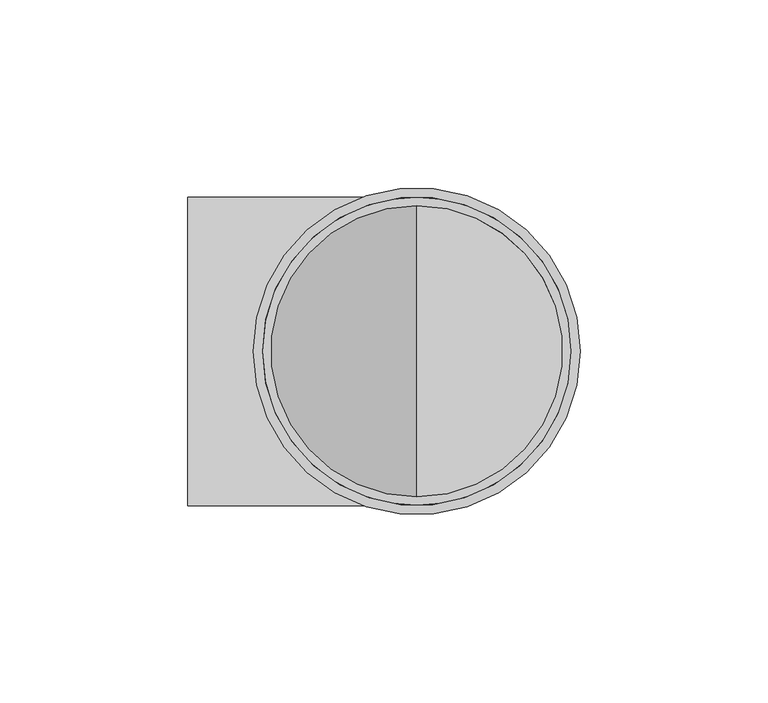
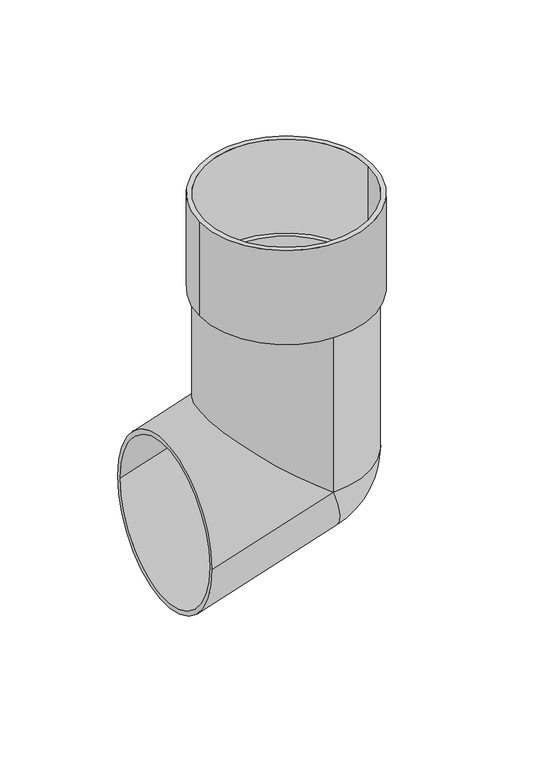
"""IFC4 building model written with IfcOpenShell, lengths in millimetres: proxy geometry, ⇲ Водосточный слив с хомутом крепления трубы : ⇲ Водосточный слив с хомутом крепления трубы."""

import ifcopenshell
import ifcopenshell.guid

model = None  # the IFC model being written
_history = None  # IfcOwnerHistory: only IFC2X3 demands one
_inside = {}  # id of a spatial element -> (the spatial element, [elements in it])
_under = {}  # id of a project, library or spatial element -> (it, [spatial elements below it])
_declared = {}  # id of a project -> (the project, [libraries it declares])
_typed = {}  # id of a type object -> (the type object, [elements of that type])
_made_of = {}  # id of a material, layer set ... -> (it, [elements and type objects made of it])


def new_model(schema):
    """Start an empty IFC model of exactly this schema.

    Asked for "IFC4X3", IfcOpenShell would pick the latest addendum, in which some entities
    have other attributes; the version numbers below select the first issue.
    IFC2X3 requires an IfcOwnerHistory on every rooted entity: one is made here for all.
    """
    global model, _history
    if schema == "IFC4X3":
        model = ifcopenshell.file(schema_version=(4, 3, 0, 0))
    else:
        model = ifcopenshell.file(schema=schema)
    _inside.clear()
    _under.clear()
    _declared.clear()
    _typed.clear()
    _made_of.clear()
    _history = None
    if model.schema == "IFC2X3":
        org = make("IfcOrganization", Name="unknown")
        user = make(
            "IfcPersonAndOrganization",
            ThePerson=make("IfcPerson", FamilyName="unknown"),
            TheOrganization=org,
        )
        app = make(
            "IfcApplication",
            ApplicationDeveloper=org,
            Version="unknown",
            ApplicationFullName="unknown",
            ApplicationIdentifier="unknown",
        )
        _history = make(
            "IfcOwnerHistory",
            OwningUser=user,
            OwningApplication=app,
            ChangeAction="ADDED",
            CreationDate=0,
        )
    return model


def make(cls, **values):
    """One entity of the class cls with the attributes given. An attribute that is None is left unset."""
    return model.create_entity(
        cls, **{name: value for name, value in values.items() if value is not None}
    )


def rooted(cls, **values):
    """An entity with a GlobalId (a new one), such as an element, a storey or a relation."""
    return make(cls, GlobalId=ifcopenshell.guid.new(), OwnerHistory=_history, **values)


def si_unit(unit_type, name, prefix=None):
    """IfcSIUnit, for example si_unit("LENGTHUNIT", "METRE", prefix="MILLI")."""
    return make("IfcSIUnit", UnitType=unit_type, Prefix=prefix, Name=name)


def assignment(units):
    """IfcUnitAssignment: the units of a project."""
    return None if units is None else make("IfcUnitAssignment", Units=units)


def point(xyz):
    """IfcCartesianPoint."""
    return None if xyz is None else make("IfcCartesianPoint", Coordinates=xyz)


def direction(xyz):
    """IfcDirection."""
    return None if xyz is None else make("IfcDirection", DirectionRatios=xyz)


def frame(location, z_axis=None, x_axis=None):
    """IfcAxis2Placement3D, a coordinate frame: its origin and axes. An axis left out is left unset."""
    return make(
        "IfcAxis2Placement3D",
        Location=point(location),
        Axis=direction(z_axis),
        RefDirection=direction(x_axis),
    )


def origin():
    """The frame at (0, 0, 0) with its axes left unset."""
    return frame((0.0, 0.0, 0.0))


def origin_with_axes():
    """The frame at (0, 0, 0) with the z axis (0, 0, 1) and the x axis (1, 0, 0) written out."""
    return frame((0.0, 0.0, 0.0), z_axis=(0.0, 0.0, 1.0), x_axis=(1.0, 0.0, 0.0))


def place(relative_to, where):
    """IfcLocalPlacement: puts the frame where relative to a parent placement (None: the world)."""
    return make(
        "IfcLocalPlacement", PlacementRelTo=relative_to, RelativePlacement=where
    )


def context(
    kind, dimensions, precision=None, world=None, true_north=None, identifier=None
):
    """IfcGeometricRepresentationContext, for example the 3D "Model" context."""
    return make(
        "IfcGeometricRepresentationContext",
        ContextIdentifier=identifier,
        ContextType=kind,
        CoordinateSpaceDimension=dimensions,
        Precision=precision,
        WorldCoordinateSystem=world,
        TrueNorth=true_north,
    )


def project(units=None, contexts=None):
    """IfcProject with its units and contexts."""
    return rooted(
        "IfcProject",
        Name="project",
        RepresentationContexts=contexts,
        UnitsInContext=assignment(units),
    )


def spatial(cls, under=None, at=None, **own):
    """A site, building, storey or space (cls), placed at a placement, below another one or the project."""
    s = rooted(cls, ObjectPlacement=at, **own)
    if under is not None:
        _under.setdefault(under.id(), (under, []))[1].append(s)
    return s


def polyline(points):
    """IfcPolyline through the points."""
    return make("IfcPolyline", Points=[point(p) for p in points])


def circle_curve(where, radius):
    """IfcCircle in the frame where."""
    return make("IfcCircle", Position=where, Radius=radius)


def ellipse_curve(where, semi_axis1, semi_axis2):
    """IfcEllipse in the frame where."""
    return make(
        "IfcEllipse", Position=where, SemiAxis1=semi_axis1, SemiAxis2=semi_axis2
    )


def trimmed(basis, trim1, trim2, sense, master):
    """IfcTrimmedCurve: the piece of a basis curve between two trims."""
    return make(
        "IfcTrimmedCurve",
        BasisCurve=basis,
        Trim1=trim1,
        Trim2=trim2,
        SenseAgreement=sense,
        MasterRepresentation=master,
    )


def shape(context_of_items, identifier, shape_type, items):
    """IfcShapeRepresentation: the items that make up one representation, for example the "Body"."""
    return make(
        "IfcShapeRepresentation",
        ContextOfItems=context_of_items,
        RepresentationIdentifier=identifier,
        RepresentationType=shape_type,
        Items=items,
    )


def source(mapping_origin, context_of_items, identifier, shape_type, items):
    """IfcRepresentationMap: a shape defined once, which mapped items show again and again."""
    return make(
        "IfcRepresentationMap",
        MappingOrigin=mapping_origin,
        MappedRepresentation=shape(context_of_items, identifier, shape_type, items),
    )


def transform(
    local_origin,
    x_axis=None,
    y_axis=None,
    z_axis=None,
    scale=None,
    scale2=None,
    scale3=None,
    uniform=True,
):
    """IfcCartesianTransformationOperator3D, or its non-uniform kind. x_axis, y_axis, z_axis: its Axis1, 2, 3."""
    if uniform:
        return make(
            "IfcCartesianTransformationOperator3D",
            Axis1=direction(x_axis),
            Axis2=direction(y_axis),
            LocalOrigin=point(local_origin),
            Scale=scale,
            Axis3=direction(z_axis),
        )
    return make(
        "IfcCartesianTransformationOperator3DnonUniform",
        Axis1=direction(x_axis),
        Axis2=direction(y_axis),
        LocalOrigin=point(local_origin),
        Scale=scale,
        Axis3=direction(z_axis),
        Scale2=scale2,
        Scale3=scale3,
    )


def mapped(mapping_source, mapping_target):
    """IfcMappedItem: shows the shape of a source again, moved by a transform."""
    return make(
        "IfcMappedItem", MappingSource=mapping_source, MappingTarget=mapping_target
    )


def made_of(thing, what):
    """Note that an element or type object is made of a material, layer set ...; save() writes the relation."""
    if what is not None:
        _made_of.setdefault(what.id(), (what, []))[1].append(thing)
    return thing


def element(
    cls,
    number,
    at=None,
    inside=None,
    cuts=None,
    type_object=None,
    material=None,
    context=None,
    identifier="Body",
    shape_type=None,
    held_by="IfcProductDefinitionShape",
    body=None,
    shapes=None,
    **own,
):
    """One element of the class cls, such as IfcWall. Its Tag is "e" and its number.

    at: its placement. inside: the storey or other place that contains it. cuts: it is an
    opening in that element (IfcRelVoidsElement). A single representation is given by context,
    identifier, shape_type and body (its items); several are given by shapes. held_by: the class
    of the entity that holds the representations. save() writes the other relations.
    """
    e = rooted(cls, Tag="e%d" % number, ObjectPlacement=at, **own)
    if body is not None:
        shapes = [shape(context, identifier, shape_type, body)]
    if shapes is not None:
        e.Representation = make(held_by, Representations=shapes)
    if inside is not None:
        _inside.setdefault(inside.id(), (inside, []))[1].append(e)
    if cuts is not None:
        rooted(
            "IfcRelVoidsElement", RelatingBuildingElement=cuts, RelatedOpeningElement=e
        )
    if type_object is not None:
        _typed.setdefault(type_object.id(), (type_object, []))[1].append(e)
    return made_of(e, material)


def aggregate(whole, parts):
    """IfcRelAggregates: a whole, such as a stair, and the parts it consists of."""
    return rooted("IfcRelAggregates", RelatingObject=whole, RelatedObjects=parts)


def save(model, path):
    """Write the relations noted so far, then the file.

    IfcRelAggregates (storeys below a building ...), IfcRelContainedInSpatialStructure (elements
    in a storey), IfcRelDefinesByType, IfcRelAssociatesMaterial and IfcRelDeclares: one each for
    every whole, place, type object, material and project.
    """
    for whole, parts in _under.values():
        aggregate(whole, parts)
    for where, things in _inside.values():
        rooted(
            "IfcRelContainedInSpatialStructure",
            RelatedElements=things,
            RelatingStructure=where,
        )
    for kind, things in _typed.values():
        rooted("IfcRelDefinesByType", RelatedObjects=things, RelatingType=kind)
    for what, things in _made_of.values():
        rooted("IfcRelAssociatesMaterial", RelatedObjects=things, RelatingMaterial=what)
    for by, libraries in _declared.values():
        rooted("IfcRelDeclares", RelatingContext=by, RelatedDefinitions=libraries)
    model.write(path)


def plane_surface(at):
    """IfcPlane: the flat surface through the origin of the frame at, square to its z axis."""
    return make("IfcPlane", Position=at)


def cylinder_surface(at, radius):
    """IfcCylindricalSurface: all points at the distance radius from the z axis of the frame at."""
    return make("IfcCylindricalSurface", Position=at, Radius=radius)


def revolved_surface(curve, axis_point, axis_direction):
    """IfcSurfaceOfRevolution: the curve turned about the line through axis_point along axis_direction."""
    return make(
        "IfcSurfaceOfRevolution",
        SweptCurve=make("IfcArbitraryOpenProfileDef", ProfileType="CURVE", Curve=curve),
        AxisPosition=make("IfcAxis1Placement", Location=point(axis_point), Axis=direction(axis_direction)),
    )


def advanced_brep(points, edges, surfaces, faces):
    """IfcAdvancedBrep: a solid bounded by faces that lie on surfaces and meet in shared edges.

    An edge is (start, end): straight between two places in points (the first is 0);
    or (start, end, curve); or (start, end, curve, False) where it runs against its curve.
    A face is (place in surfaces, loops), or (place, loops, False) where it looks against
    its surface's normal. A loop lists edges by number (the first is 1), with a minus sign
    where the edge is run from its end to its start. The first loop is the outer one.
    """
    corners = [point(p) for p in points]
    vertices = [make("IfcVertexPoint", VertexGeometry=c) for c in corners]
    made = []
    for start, end, *more in edges:
        made.append(
            make(
                "IfcEdgeCurve",
                EdgeStart=vertices[start],
                EdgeEnd=vertices[end],
                EdgeGeometry=more[0] if more else make("IfcPolyline", Points=[corners[start], corners[end]]),
                SameSense=more[1] if len(more) > 1 else True,
            )
        )
    hull = []
    for where, loops, *sense in faces:
        bounds = []
        for j, loop in enumerate(loops):
            ring = [make("IfcOrientedEdge", EdgeElement=made[abs(k) - 1], Orientation=k > 0) for k in loop]
            bounds.append(
                make(
                    "IfcFaceOuterBound" if j == 0 else "IfcFaceBound",
                    Bound=make("IfcEdgeLoop", EdgeList=ring),
                    Orientation=True,
                )
            )
        hull.append(make("IfcAdvancedFace", Bounds=bounds, FaceSurface=surfaces[where], SameSense=sense[0] if sense else True))
    return make("IfcAdvancedBrep", Outer=make("IfcClosedShell", CfsFaces=hull))


def generic_models_fbe01fe8(model_context):
    return source(origin(), model_context, "Body", "AdvancedBrep", [
        advanced_brep(
        [(41.1, 0.0, -50.0), (0.0, 41.1, -50.0), (-41.1, 0.0, -50.0), (0.0, -41.1, -50.0), (0.0, 38.8, -50.0), (0.0, -38.8, -50.0), (0.0, 41.1, -50.0), (0.0, 41.1, -134.0), (0.0, -41.1, -134.0), (0.0, -41.1, -50.0), (-41.1, 0.0, -50.0), (41.1, 0.0, -50.0), (0.0, 38.8, -134.0), (0.0, -38.8, -134.0), (-61.0, 41.1, -153.8201015), (-61.0, -41.1, -153.8201015), (-61.0, 38.8, -153.8201015), (-61.0, -38.8, -153.8201015), (-43.6, 0.0, 0.0), (43.6, 0.0, 0.0), (-41.1, 0.0, 0.0), (41.1, 0.0, 0.0), (-43.6, 0.0, -50.0), (43.6, 0.0, -50.0)],
        [
            (0, 1, circle_curve(frame((0.0, 0.0, -50.0), z_axis=(0.0, 0.0, 1.0), x_axis=(1.0, 0.0, 0.0)), 41.1)),
            (1, 2, circle_curve(frame((0.0, 0.0, -50.0), z_axis=(0.0, 0.0, 1.0), x_axis=(1.0, 0.0, 0.0)), 41.1)),
            (2, 3, circle_curve(frame((0.0, 0.0, -50.0), z_axis=(0.0, 0.0, 1.0), x_axis=(1.0, 0.0, 0.0)), 41.1)),
            (3, 0, circle_curve(frame((0.0, 0.0, -50.0), z_axis=(0.0, 0.0, 1.0), x_axis=(1.0, 0.0, 0.0)), 41.1)),
            (4, 5, circle_curve(frame((0.0, 0.0, -50.0), z_axis=(0.0, 0.0, -1.0), x_axis=(0.0, -1.0, 0.0)), 38.8)),
            (5, 4, circle_curve(frame((0.0, 0.0, -50.0), z_axis=(0.0, 0.0, -1.0), x_axis=(0.0, -1.0, 0.0)), 38.8)),
            (6, 7),
            (7, 8, ellipse_curve(frame((0.0, 0.0, -134.0), z_axis=(0.5877852522924744, 0.0, 0.8090169943749465), x_axis=(-0.8090169943749465, 0.0, 0.5877852522924745)), 50.8023939, 41.1)),
            (8, 9),
            (9, 10, circle_curve(frame((0.0, 0.0, -50.0), z_axis=(0.0, 0.0, -1.0), x_axis=(0.0, -1.0, 0.0)), 41.1)),
            (10, 6, circle_curve(frame((0.0, 0.0, -50.0), z_axis=(0.0, 0.0, -1.0), x_axis=(0.0, -1.0, 0.0)), 41.1)),
            (6, 11, circle_curve(frame((0.0, 0.0, -50.0), z_axis=(0.0, 0.0, -1.0), x_axis=(0.0, -1.0, 0.0)), 41.1)),
            (11, 9, circle_curve(frame((0.0, 0.0, -50.0), z_axis=(0.0, 0.0, -1.0), x_axis=(0.0, -1.0, 0.0)), 41.1)),
            (8, 7, circle_curve(frame((0.0, 0.0, -134.0), z_axis=(0.0, 0.0, 1.0), x_axis=(0.0, -1.0, 0.0)), 41.1)),
            (4, 12),
            (12, 13, circle_curve(frame((0.0, 0.0, -134.0), z_axis=(0.0, 0.0, -1.0), x_axis=(0.0, -1.0, 0.0)), 38.8)),
            (13, 5),
            (13, 12, ellipse_curve(frame((0.0, 0.0, -134.0), z_axis=(-0.5877852522924744, 0.0, -0.8090169943749465), x_axis=(0.8090169943749465, 0.0, -0.5877852522924745)), 47.9594375, 38.8)),
            (7, 14),
            (14, 15, ellipse_curve(frame((-61.0, 0.0, -153.8201015), z_axis=(1.0, 0.0, 0.0), x_axis=(0.0, 0.0, 1.0)), 43.2150974, 41.1)),
            (15, 8),
            (7, 8, circle_curve(frame((0.0, 0.0, -134.0), z_axis=(-0.9510565162951546, 0.0, -0.30901699437494456), x_axis=(0.0, -1.0, 0.0)), 41.1)),
            (15, 14, ellipse_curve(frame((-61.0, 0.0, -153.8201015), z_axis=(1.0, 0.0, 0.0), x_axis=(0.0, 0.0, 1.0)), 43.2150974, 41.1)),
            (13, 12, circle_curve(frame((0.0, 0.0, -134.0), z_axis=(0.9510565162951546, 0.0, 0.30901699437494456), x_axis=(0.0, -1.0, 0.0)), 38.8)),
            (12, 16),
            (16, 17, ellipse_curve(frame((-61.0, 0.0, -153.8201015), z_axis=(-1.0, 0.0, 0.0), x_axis=(0.0, 0.0, -1.0)), 40.7967343, 38.8)),
            (17, 13),
            (17, 16, ellipse_curve(frame((-61.0, 0.0, -153.8201015), z_axis=(-1.0, 0.0, 0.0), x_axis=(0.0, 0.0, -1.0)), 40.7967343, 38.8)),
            (12, 13),
            (18, 19, circle_curve(origin_with_axes(), 43.6)),
            (19, 18, circle_curve(origin_with_axes(), 43.6)),
            (20, 21, circle_curve(frame((0.0, 0.0, 0.0), z_axis=(0.0, 0.0, -1.0), x_axis=(1.0, 0.0, 0.0)), 41.1)),
            (21, 20, circle_curve(frame((0.0, 0.0, 0.0), z_axis=(0.0, 0.0, -1.0), x_axis=(1.0, 0.0, 0.0)), 41.1)),
            (22, 23, circle_curve(frame((0.0, 0.0, -50.0), z_axis=(0.0, 0.0, -1.0), x_axis=(1.0, 0.0, 0.0)), 43.6)),
            (23, 22, circle_curve(frame((0.0, 0.0, -50.0), z_axis=(0.0, 0.0, -1.0), x_axis=(1.0, 0.0, 0.0)), 43.6)),
            (20, 2),
            (0, 21),
            (18, 22),
            (23, 19),
        ],
        [
            plane_surface(frame((0.0, 0.0, -50.0), z_axis=(0.0, 0.0, 1.0), x_axis=(0.0, -1.0, 0.0))),
            cylinder_surface(frame((0.0, 0.0, -50.0), z_axis=(0.0, 0.0, 1.0), x_axis=(0.0, -1.0, 0.0)), 41.1),
            revolved_surface(polyline([(0.0, -38.8, -134.0), (0.0, -38.8, -50.0)]), (0.0, 0.0, -50.0), (0.0, 0.0, -1.0)),
            revolved_surface(polyline([(0.0, -38.8, -162.18985007074266), (0.0, -38.8, -50.0)]), (0.0, 0.0, -50.0), (0.0, 0.0, -1.0)),
            cylinder_surface(frame((0.0, 0.0, -134.0), z_axis=(0.9510565162951546, 0.0, 0.30901699437494456), x_axis=(0.0, -1.0, 0.0)), 41.1),
            revolved_surface(polyline([(-72.98985939037308, -38.8, -157.7158429412023), (0.0, -38.8, -134.0)]), (0.0, 0.0, -134.0), (-0.9510565162951546, 0.0, -0.30901699437494456)),
            revolved_surface(polyline([(-72.98985939037308, -38.8, -157.7158429412023), (26.810140603163227, -38.8, -125.28885725925879)]), (0.0, 0.0, -134.0), (-0.9510565162951546, 0.0, -0.30901699437494456)),
            plane_surface(frame((0.0, 50.0, -134.0), z_axis=(0.0, 0.0, 1.0), x_axis=(1.0, 0.0, 0.0))),
            plane_surface(frame((0.0, 50.0, -134.0), z_axis=(-0.9510565162951546, 0.0, -0.30901699437494445), x_axis=(0.30901699437494445, 0.0, -0.9510565162951546))),
            revolved_surface(trimmed(ellipse_curve(frame((0.0, 0.0, -134.0), z_axis=(0.0, 0.0, 1.0), x_axis=(1.0, 0.0, 0.0)), 41.1, 41.1), [point((0.0, -41.1, -134.0))], [point((0.0, 41.1, -134.0))], True, "CARTESIAN"), (0.0, 50.0, -134.0), (0.0, 1.0, 0.0)),
            plane_surface(frame((41.1, 0.0, 0.0), z_axis=(0.0, 0.0, 1.0), x_axis=(0.0, -1.0, 0.0))),
            plane_surface(frame((41.1, 0.0, -50.0), z_axis=(0.0, 0.0, -1.0), x_axis=(0.0, 1.0, 0.0))),
            revolved_surface(polyline([(41.1, 0.0, -50.0), (41.1, 0.0, 0.0)]), (0.0, 0.0, -50.0), (0.0, 0.0, -1.0)),
            cylinder_surface(origin_with_axes(), 43.6),
            plane_surface(frame((-61.0, -49.4498638, -215.0), z_axis=(-1.0, 0.0, 0.0), x_axis=(0.0, 1.0, 0.0))),
        ],
        [
            (0, [[1, 2, 3, 4], [5, 6]]),
            (1, [[7, 8, 9, 10, 11]]),
            (1, [[-7, 12, 13, -9, 14]]),
            (2, [[-5, 15, 16, 17]]),
            (3, [[-6, -17, 18, -15]]),
            (4, [[-8, 19, 20, 21]]),
            (4, [[22, -21, 23, -19]]),
            (5, [[24, 25, 26, 27]]),
            (6, [[-18, -27, 28, -25]]),
            (7, [[29, -16]]),
            (8, [[-29, -24]]),
            (9, [[-14, -22]]),
            (10, [[30, 31], [32, 33]]),
            (11, [[34, 35], [-11, -10, -13, -12]]),
            (12, [[-32, 36, -2, -1, 37]]),
            (12, [[-33, -37, -4, -3, -36]]),
            (13, [[-30, 38, -35, 39]]),
            (13, [[-31, -39, -34, -38]]),
            (14, [[-20, -23], [-26, -28]]),
        ],
    ),
    ])


if __name__ == "__main__":
    model = new_model("IFC4")
    model_context = context("Model", 3, world=origin())
    ifc_project = project(units=[si_unit("LENGTHUNIT", "METRE", prefix="MILLI")], contexts=[model_context])
    site = spatial("IfcSite", under=ifc_project)
    building = spatial("IfcBuilding", under=site)
    placement = place(None, origin())
    generic_models_shape = generic_models_fbe01fe8(model_context)
    element("IfcBuildingElementProxy", 1, Name="⇲ Водосточный слив с хомутом крепления трубы : ⇲ Водосточный слив с хомутом крепления трубы", ObjectType="⇲ Водосточный слив с хомутом крепления трубы : ⇲ Водосточный слив с хомутом крепления трубы", at=placement, inside=building, context=model_context, shape_type="MappedRepresentation", body=[
        mapped(generic_models_shape, transform((0.0, 0.0, 0.0), x_axis=(1.0, 0.0, 0.0), y_axis=(0.0, 1.0, 0.0), z_axis=(0.0, 0.0, 1.0))),
    ])
    save(model, "model.ifc")

# Revit data of these elements
# Type "⇲ Водосточный слив с хомутом крепления трубы : ⇲ Водосточный слив с хомутом крепления трубы"
#   Description = "Обеспечивает отвод воды из водосточной системы на землю"
#   Manufacturer = "ТехноНИКОЛЬ"
#   Model = "Комплектующие к водосточным системам"
#   URL = "https://tn-vodostok.ru/catalog/pvh/"
#   ADSK_Обозначение = "ТехноНИКОЛЬ"
#   ADSK_Наименование краткое = "Слив"
#   ADSK_Наименование = "Водосточный слив"
#   ADSK_Масса_Текст = ""
#   ADSK_Марка = ""
#   ADSK_Код изделия = ""
#   ADSK_Завод-изготовитель = "ТехноНИКОЛЬ"
#   ADSK_Единица измерения = "шт."
#   ADSK_Группирование = "Комплектующие к водосточным системам"
#   ADSK_URL страницы изделия = "https://tn-vodostok.ru/catalog/pvh/"
#   ADSK_URL документации изделия = "https://tn-vodostok.ru/upload/iblock/c42/c427963cb77eb5c3c51f0cfb870e9e52.pdf"
#   Угол поворота хомута [instance default] = 0.00°
#   ADSK_Размер_Ширина = 87.2 mm
#   ADSK_Размер_Диаметр = 82.2 mm
#   ADSK_Размер_Высота = 196.7 mm
#   ADSK_Количество = 1
#   ADSK_Материал [instance default] = TN_Пластик_Коричневый_RAL8019
#   Default Elevation = 0
# Element 1 (IfcBuildingElementProxy, "⇲ Водосточный слив с хомутом крепления трубы : ⇲ Водосточный слив с хомутом крепления трубы")
#   Materials on its faces: "TN_Пластик_Коричневый_RAL8019"
# Materials
#   "TN_Пластик_Коричневый_RAL8019": class "Типовые", colour RGB 61 54 53, transparency 0, Cost = 0
